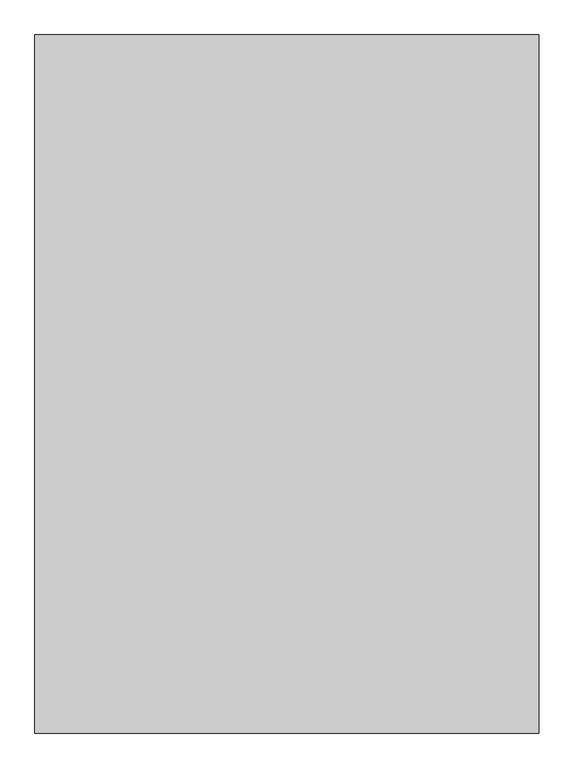
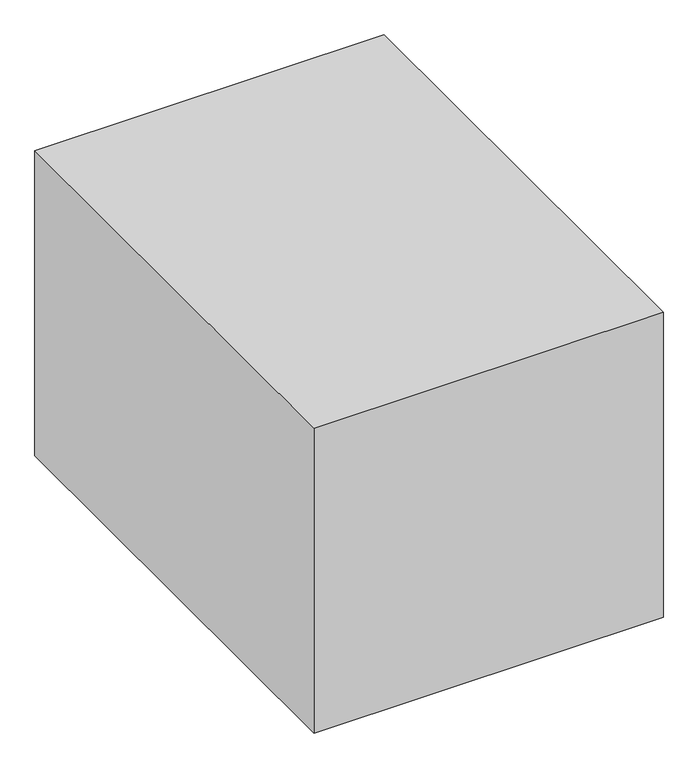
"""IFC4 building model written with IfcOpenShell, lengths in millimetres: proxy geometry, Space Planning Box_hec : Space Planning Box_hec."""

from ifc_helpers import new_model, si_unit, origin, origin_with_axes, place, context, project, spatial, polyline, outline, extrude, source, transform, mapped, element, save


def generic_models_1d705098(model_context):
    return source(origin(), model_context, "Body", "SweptSolid", [
        extrude(outline(polyline([(3250.0, 4500.0), (3250.0, -4500.0), (-3250.0, -4500.0), (-3250.0, 4500.0), (3250.0, 4500.0)])), origin_with_axes(), (0.0, 0.0, 1.0), 6000.0),
    ])


if __name__ == "__main__":
    model = new_model("IFC4")
    model_context = context("Model", 3, world=origin())
    ifc_project = project(units=[si_unit("LENGTHUNIT", "METRE", prefix="MILLI")], contexts=[model_context])
    site = spatial("IfcSite", under=ifc_project)
    building = spatial("IfcBuilding", under=site)
    placement = place(None, origin())
    generic_models_shape = generic_models_1d705098(model_context)
    element("IfcBuildingElementProxy", 1, Name="Space Planning Box_hec : Space Planning Box_hec", ObjectType="Space Planning Box_hec : Space Planning Box_hec", at=placement, inside=building, context=model_context, shape_type="MappedRepresentation", body=[
        mapped(generic_models_shape, transform((0.0, 0.0, 0.0), x_axis=(1.0, 0.0, 0.0), y_axis=(0.0, 1.0, 0.0), z_axis=(0.0, 0.0, 1.0))),
    ])
    save(model, "model.ifc")

# Revit data of these elements
# Type "Space Planning Box_hec : Space Planning Box_hec"
#   Type Comments = "..."
#   Room Name [instance default] = "?"
#   Interior Finish [instance default] = ""
#   Exterior Finish [instance default] = ""
#   Department [instance default] = ""
#   Assembly Code = "..."
#   Width [instance default] = 1524 mm
#   Program Area [instance default] = 0.00 m²
#   Length [instance default] = 1524 mm
#   Height [instance default] = 1524 mm
#   Area [instance default] = 2.32258 m²
#   Fill Color [instance default] = Cyan
#   Default Elevation = 0
# Element 1 (IfcBuildingElementProxy, "Space Planning Box_hec : Space Planning Box_hec")
#   Room Name = "Switchgear Room"
#   Interior Finish = "IF1"
#   Exterior Finish = "EF1"
#   Department = "EL"
#   Width = 6500 mm
#   Program Area = 58.50 m²
#   Length = 9000 mm
#   Height = 6000 mm
#   Area = 58.50 m²
#   Fill Color = Blue
#   Materials on its faces: "Blue"
# Materials
#   "Cyan": class "Generic", colour RGB 0 255 255, transparency 0.2, Cost = 0
#   "Blue": class "Generic", colour RGB 0 0 255, transparency 0.2, Cost = 0
